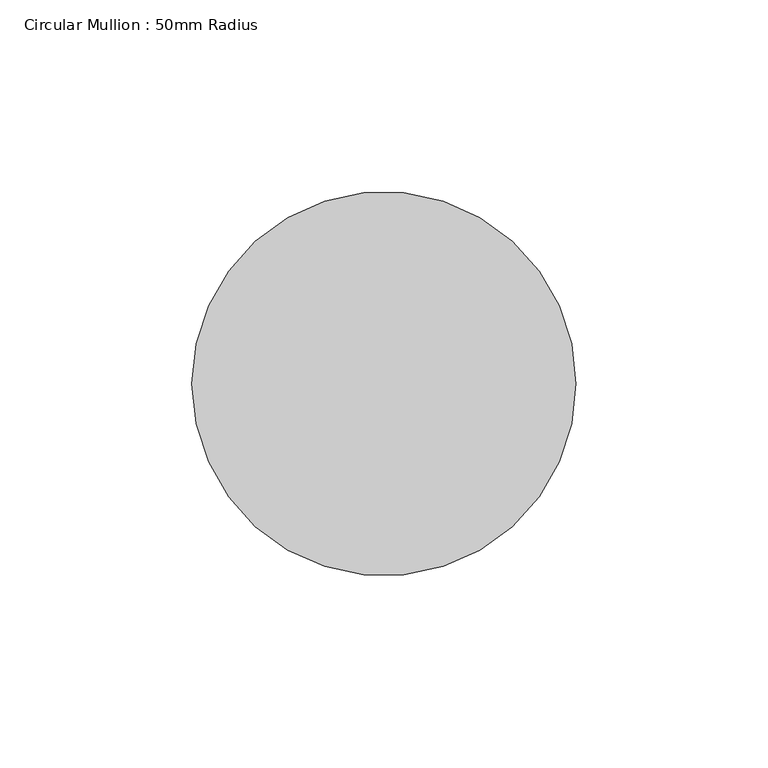
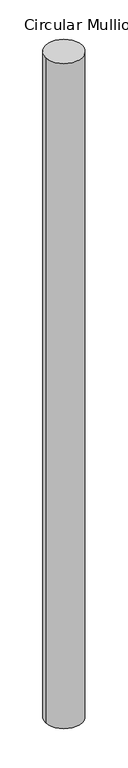
"""IFC4 building model written with IfcOpenShell, lengths in millimetres: member geometry, Circular Mullion : 50mm Radius."""

from ifc_helpers import new_model, si_unit, point, frame, frame_2d, origin, place, context, project, spatial, circle_curve, trimmed, segment, composite_curve, outline, extrude, source, transform, mapped, element, save


def circular_mullion_50mm_radius_751a37ba(model_context):
    return source(origin(), model_context, "Body", "SweptSolid", [
        extrude(outline(composite_curve([segment(trimmed(circle_curve(frame_2d((-50.0, 0.0)), 50.0), [point((0.0, 0.0))], [point((-100.0, 0.0))], False, "CARTESIAN"), True, "CONTINUOUS"), segment(trimmed(circle_curve(frame_2d((-50.0, 0.0)), 50.0), [point((-100.0, 0.0))], [point((0.0, 0.0))], False, "CARTESIAN"), True, "CONTINUOUS")], self_intersect=False)), frame((0.0, 0.0, -1915.3845628), z_axis=(0.0, 0.0, 1.0), x_axis=(1.0, 0.0, 0.0)), (0.0, 0.0, 1.0), 1915.3845628),
    ])


if __name__ == "__main__":
    model = new_model("IFC4")
    model_context = context("Model", 3, world=origin())
    ifc_project = project(units=[si_unit("LENGTHUNIT", "METRE", prefix="MILLI")], contexts=[model_context])
    site = spatial("IfcSite", under=ifc_project)
    building = spatial("IfcBuilding", under=site)
    placement = place(None, origin())
    circular_mullion_50mm_radius_shape = circular_mullion_50mm_radius_751a37ba(model_context)
    element("IfcMember", 1, ObjectType="Circular Mullion : 50mm Radius", at=placement, inside=building, context=model_context, shape_type="MappedRepresentation", body=[
        mapped(circular_mullion_50mm_radius_shape, transform((0.0, 0.0, 0.0), x_axis=(1.0, 0.0, 0.0), y_axis=(0.0, 1.0, 0.0), z_axis=(0.0, 0.0, 1.0))),
    ])
    save(model, "model.ifc")

# Revit data of these elements
# Type "Circular Mullion : 50mm Radius"
#   built-in parameter 1007350 = 0.164042 (stored number, unit not read)
# Element 1 (IfcMember, "Circular Mullion : 50mm Radius")
#   Materials on its faces: "Aluminium"
# Materials
#   "Aluminium": class "Metal", colour RGB 247 247 247, transparency 0, Description = "Aluminium 6061", Cost = 0
